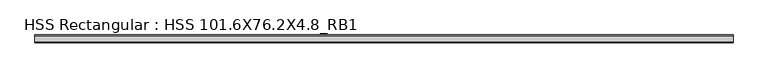
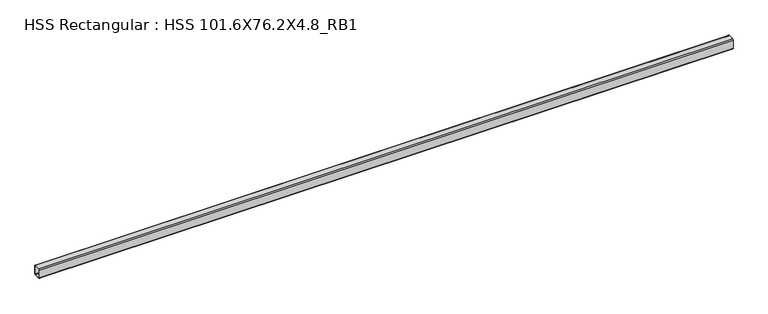
"""IFC4 building model written with IfcOpenShell, lengths in millimetres: beam geometry, HSS Rectangular : HSS 101.6X76.2X4.8_RB1."""

from ifc_helpers import new_model, si_unit, point, frame, frame_2d, origin, place, context, project, spatial, polyline, circle_curve, trimmed, segment, composite_curve, outline, extrude, source, transform, mapped, element, save


def hss_rectangular_hss_101_6x76_2x4_8_rb1_618717bd(model_context):
    return source(origin(), model_context, "Body", "SweptSolid", [
        extrude(outline(composite_curve([segment(polyline([(38.1, 41.275), (38.1, -41.275)]), True, "CONTINUOUS"), segment(trimmed(circle_curve(frame_2d((28.575, -41.275)), 9.525), [point((38.1, -41.275))], [point((28.575, -50.8))], False, "CARTESIAN"), True, "CONTINUOUS"), segment(polyline([(28.575, -50.8), (-28.575, -50.8)]), True, "CONTINUOUS"), segment(trimmed(circle_curve(frame_2d((-28.575, -41.275)), 9.525), [point((-28.575, -50.8))], [point((-38.1, -41.275))], False, "CARTESIAN"), True, "CONTINUOUS"), segment(polyline([(-38.1, -41.275), (-38.1, 41.275)]), True, "CONTINUOUS"), segment(trimmed(circle_curve(frame_2d((-28.575, 41.275)), 9.525), [point((-38.1, 41.275))], [point((-28.575, 50.8))], False, "CARTESIAN"), True, "CONTINUOUS"), segment(polyline([(-28.575, 50.8), (28.575, 50.8)]), True, "CONTINUOUS"), segment(trimmed(circle_curve(frame_2d((28.575, 41.275)), 9.525), [point((28.575, 50.8))], [point((38.1, 41.275))], False, "CARTESIAN"), True, "CONTINUOUS")], self_intersect=False), holes=[composite_curve([segment(trimmed(circle_curve(frame_2d((-28.575, 41.275)), 4.7625), [point((-28.575, 46.0375))], [point((-33.3375, 41.275))], True, "CARTESIAN"), True, "CONTINUOUS"), segment(polyline([(-33.3375, 41.275), (-33.3375, -41.275)]), True, "CONTINUOUS"), segment(trimmed(circle_curve(frame_2d((-28.575, -41.275)), 4.7625), [point((-33.3375, -41.275))], [point((-28.575, -46.0375))], True, "CARTESIAN"), True, "CONTINUOUS"), segment(polyline([(-28.575, -46.0375), (28.575, -46.0375)]), True, "CONTINUOUS"), segment(trimmed(circle_curve(frame_2d((28.575, -41.275)), 4.7625), [point((28.575, -46.0375))], [point((33.3375, -41.275))], True, "CARTESIAN"), True, "CONTINUOUS"), segment(polyline([(33.3375, -41.275), (33.3375, 41.275)]), True, "CONTINUOUS"), segment(trimmed(circle_curve(frame_2d((28.575, 41.275)), 4.7625), [point((33.3375, 41.275))], [point((28.575, 46.0375))], True, "CARTESIAN"), True, "CONTINUOUS"), segment(polyline([(28.575, 46.0375), (-28.575, 46.0375)]), True, "CONTINUOUS")], self_intersect=False)]), frame((1171.1784188, 0.0, 0.0), z_axis=(1.0, 0.0, 0.0), x_axis=(0.0, 1.0, 0.0)), (0.0, 0.0, 1.0), 6796.0923551),
    ])


if __name__ == "__main__":
    model = new_model("IFC4")
    model_context = context("Model", 3, world=origin())
    ifc_project = project(units=[si_unit("LENGTHUNIT", "METRE", prefix="MILLI")], contexts=[model_context])
    site = spatial("IfcSite", under=ifc_project)
    building = spatial("IfcBuilding", under=site)
    placement = place(None, origin())
    hss_rectangular_hss_101_6x76_2x4_8_rb1_shape = hss_rectangular_hss_101_6x76_2x4_8_rb1_618717bd(model_context)
    element("IfcBeam", 1, ObjectType="HSS Rectangular : HSS 101.6X76.2X4.8_RB1", at=placement, inside=building, context=model_context, shape_type="MappedRepresentation", body=[
        mapped(hss_rectangular_hss_101_6x76_2x4_8_rb1_shape, transform((0.0, 0.0, 0.0), x_axis=(1.0, 0.0, 0.0), y_axis=(0.0, 1.0, 0.0), z_axis=(0.0, 0.0, 1.0))),
    ])
    save(model, "model.ifc")

# Revit data of these elements
# Type "HSS Rectangular : HSS 101.6X76.2X4.8_RB1"
#   Section Name Key = "HSS 4X3X3/16"
#   Assembly Code = "B10"
#   Width = 7.62 cm
#   Wall Nominal Thickness = 0.4763 cm
#   Wall Design Thickness = 0.442 cm
#   Torsional Moment of Inertia = 260.561 cm⁴
#   Torsional Modulus = 61.2876 cm³
#   Section Area = 14.4516 cm²
#   Plastic Modulus weak axis = 40.3122 cm³
#   Plastic Modulus strong axis = 49.1612 cm³
#   Perimeter = 0.881482 m²/m
#   Outer Fillet = 0.9525 cm
#   Nominal Weight = 12.1285 kgf/m
#   Moment of Inertia weak axis = 131.529 cm⁴
#   Moment of Inertia strong axis = 205.202 cm⁴
#   Inner Fillet = 0.4763 cm
#   Height = 10.16 cm
#   Elastic Modulus weak axis = 34.4128 cm³
#   Elastic Modulus strong axis = 40.476 cm³
#   Centroid Vertical = 5.08 cm
#   Centroid Horizontal = 3.81 cm
#   Length [instance default] = 1524 mm
#   Structural Material [instance default] = Steel ASTM A500, Grade B, Rectangular and Square
#   Principal Axes Angle = 0
# Element 1 (IfcBeam, "HSS Rectangular : HSS 101.6X76.2X4.8_RB1")
#   Structural Material = Steel ASTM A992
#   Materials on its faces: "Steel ASTM A992"
# Materials
#   "Steel ASTM A500, Grade B, Rectangular and Square": class "Metal", colour RGB 199 199 199, transparency 0, Description = "Carbon steel", Cost = 0
#   "Steel ASTM A992": class "Metal", colour RGB 199 199 199, transparency 0, Description = "Structural steel 50ksi", Cost = 0
